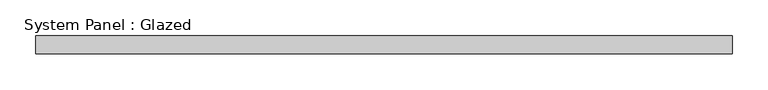
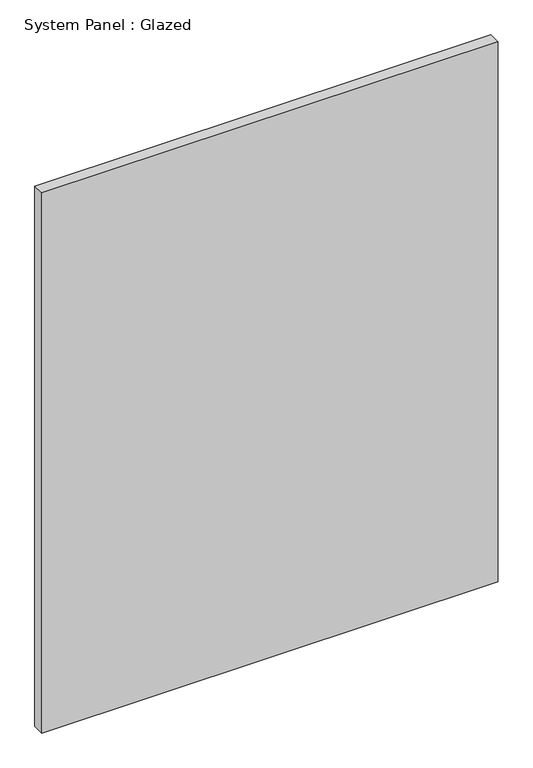
"""IFC4 building model written with IfcOpenShell, lengths in millimetres: plate geometry, System Panel : Glazed."""

import ifcopenshell
import ifcopenshell.guid

model = None  # the IFC model being written
_history = None  # IfcOwnerHistory: only IFC2X3 demands one
_inside = {}  # id of a spatial element -> (the spatial element, [elements in it])
_under = {}  # id of a project, library or spatial element -> (it, [spatial elements below it])
_declared = {}  # id of a project -> (the project, [libraries it declares])
_typed = {}  # id of a type object -> (the type object, [elements of that type])
_made_of = {}  # id of a material, layer set ... -> (it, [elements and type objects made of it])


def new_model(schema):
    """Start an empty IFC model of exactly this schema.

    Asked for "IFC4X3", IfcOpenShell would pick the latest addendum, in which some entities
    have other attributes; the version numbers below select the first issue.
    IFC2X3 requires an IfcOwnerHistory on every rooted entity: one is made here for all.
    """
    global model, _history
    if schema == "IFC4X3":
        model = ifcopenshell.file(schema_version=(4, 3, 0, 0))
    else:
        model = ifcopenshell.file(schema=schema)
    _inside.clear()
    _under.clear()
    _declared.clear()
    _typed.clear()
    _made_of.clear()
    _history = None
    if model.schema == "IFC2X3":
        org = make("IfcOrganization", Name="unknown")
        user = make(
            "IfcPersonAndOrganization",
            ThePerson=make("IfcPerson", FamilyName="unknown"),
            TheOrganization=org,
        )
        app = make(
            "IfcApplication",
            ApplicationDeveloper=org,
            Version="unknown",
            ApplicationFullName="unknown",
            ApplicationIdentifier="unknown",
        )
        _history = make(
            "IfcOwnerHistory",
            OwningUser=user,
            OwningApplication=app,
            ChangeAction="ADDED",
            CreationDate=0,
        )
    return model


def make(cls, **values):
    """One entity of the class cls with the attributes given. An attribute that is None is left unset."""
    return model.create_entity(
        cls, **{name: value for name, value in values.items() if value is not None}
    )


def rooted(cls, **values):
    """An entity with a GlobalId (a new one), such as an element, a storey or a relation."""
    return make(cls, GlobalId=ifcopenshell.guid.new(), OwnerHistory=_history, **values)


def si_unit(unit_type, name, prefix=None):
    """IfcSIUnit, for example si_unit("LENGTHUNIT", "METRE", prefix="MILLI")."""
    return make("IfcSIUnit", UnitType=unit_type, Prefix=prefix, Name=name)


def assignment(units):
    """IfcUnitAssignment: the units of a project."""
    return None if units is None else make("IfcUnitAssignment", Units=units)


def point(xyz):
    """IfcCartesianPoint."""
    return None if xyz is None else make("IfcCartesianPoint", Coordinates=xyz)


def direction(xyz):
    """IfcDirection."""
    return None if xyz is None else make("IfcDirection", DirectionRatios=xyz)


def frame(location, z_axis=None, x_axis=None):
    """IfcAxis2Placement3D, a coordinate frame: its origin and axes. An axis left out is left unset."""
    return make(
        "IfcAxis2Placement3D",
        Location=point(location),
        Axis=direction(z_axis),
        RefDirection=direction(x_axis),
    )


def origin():
    """The frame at (0, 0, 0) with its axes left unset."""
    return frame((0.0, 0.0, 0.0))


def origin_with_axes():
    """The frame at (0, 0, 0) with the z axis (0, 0, 1) and the x axis (1, 0, 0) written out."""
    return frame((0.0, 0.0, 0.0), z_axis=(0.0, 0.0, 1.0), x_axis=(1.0, 0.0, 0.0))


def place(relative_to, where):
    """IfcLocalPlacement: puts the frame where relative to a parent placement (None: the world)."""
    return make(
        "IfcLocalPlacement", PlacementRelTo=relative_to, RelativePlacement=where
    )


def context(
    kind, dimensions, precision=None, world=None, true_north=None, identifier=None
):
    """IfcGeometricRepresentationContext, for example the 3D "Model" context."""
    return make(
        "IfcGeometricRepresentationContext",
        ContextIdentifier=identifier,
        ContextType=kind,
        CoordinateSpaceDimension=dimensions,
        Precision=precision,
        WorldCoordinateSystem=world,
        TrueNorth=true_north,
    )


def project(units=None, contexts=None):
    """IfcProject with its units and contexts."""
    return rooted(
        "IfcProject",
        Name="project",
        RepresentationContexts=contexts,
        UnitsInContext=assignment(units),
    )


def spatial(cls, under=None, at=None, **own):
    """A site, building, storey or space (cls), placed at a placement, below another one or the project."""
    s = rooted(cls, ObjectPlacement=at, **own)
    if under is not None:
        _under.setdefault(under.id(), (under, []))[1].append(s)
    return s


def polyline(points):
    """IfcPolyline through the points."""
    return make("IfcPolyline", Points=[point(p) for p in points])


def outline(outer, holes=None, kind="AREA"):
    """IfcArbitraryClosedProfileDef: a profile drawn as a closed curve; with holes, ...WithVoids."""
    if holes is None:
        return make("IfcArbitraryClosedProfileDef", ProfileType=kind, OuterCurve=outer)
    return make(
        "IfcArbitraryProfileDefWithVoids",
        ProfileType=kind,
        OuterCurve=outer,
        InnerCurves=holes,
    )


def extrude(swept, where, along, depth):
    """IfcExtrudedAreaSolid: the profile swept, set in the frame where, extruded along a direction by depth."""
    return make(
        "IfcExtrudedAreaSolid",
        SweptArea=swept,
        Position=where,
        ExtrudedDirection=direction(along),
        Depth=depth,
    )


def shape(context_of_items, identifier, shape_type, items):
    """IfcShapeRepresentation: the items that make up one representation, for example the "Body"."""
    return make(
        "IfcShapeRepresentation",
        ContextOfItems=context_of_items,
        RepresentationIdentifier=identifier,
        RepresentationType=shape_type,
        Items=items,
    )


def source(mapping_origin, context_of_items, identifier, shape_type, items):
    """IfcRepresentationMap: a shape defined once, which mapped items show again and again."""
    return make(
        "IfcRepresentationMap",
        MappingOrigin=mapping_origin,
        MappedRepresentation=shape(context_of_items, identifier, shape_type, items),
    )


def transform(
    local_origin,
    x_axis=None,
    y_axis=None,
    z_axis=None,
    scale=None,
    scale2=None,
    scale3=None,
    uniform=True,
):
    """IfcCartesianTransformationOperator3D, or its non-uniform kind. x_axis, y_axis, z_axis: its Axis1, 2, 3."""
    if uniform:
        return make(
            "IfcCartesianTransformationOperator3D",
            Axis1=direction(x_axis),
            Axis2=direction(y_axis),
            LocalOrigin=point(local_origin),
            Scale=scale,
            Axis3=direction(z_axis),
        )
    return make(
        "IfcCartesianTransformationOperator3DnonUniform",
        Axis1=direction(x_axis),
        Axis2=direction(y_axis),
        LocalOrigin=point(local_origin),
        Scale=scale,
        Axis3=direction(z_axis),
        Scale2=scale2,
        Scale3=scale3,
    )


def mapped(mapping_source, mapping_target):
    """IfcMappedItem: shows the shape of a source again, moved by a transform."""
    return make(
        "IfcMappedItem", MappingSource=mapping_source, MappingTarget=mapping_target
    )


def made_of(thing, what):
    """Note that an element or type object is made of a material, layer set ...; save() writes the relation."""
    if what is not None:
        _made_of.setdefault(what.id(), (what, []))[1].append(thing)
    return thing


def element(
    cls,
    number,
    at=None,
    inside=None,
    cuts=None,
    type_object=None,
    material=None,
    context=None,
    identifier="Body",
    shape_type=None,
    held_by="IfcProductDefinitionShape",
    body=None,
    shapes=None,
    **own,
):
    """One element of the class cls, such as IfcWall. Its Tag is "e" and its number.

    at: its placement. inside: the storey or other place that contains it. cuts: it is an
    opening in that element (IfcRelVoidsElement). A single representation is given by context,
    identifier, shape_type and body (its items); several are given by shapes. held_by: the class
    of the entity that holds the representations. save() writes the other relations.
    """
    e = rooted(cls, Tag="e%d" % number, ObjectPlacement=at, **own)
    if body is not None:
        shapes = [shape(context, identifier, shape_type, body)]
    if shapes is not None:
        e.Representation = make(held_by, Representations=shapes)
    if inside is not None:
        _inside.setdefault(inside.id(), (inside, []))[1].append(e)
    if cuts is not None:
        rooted(
            "IfcRelVoidsElement", RelatingBuildingElement=cuts, RelatedOpeningElement=e
        )
    if type_object is not None:
        _typed.setdefault(type_object.id(), (type_object, []))[1].append(e)
    return made_of(e, material)


def aggregate(whole, parts):
    """IfcRelAggregates: a whole, such as a stair, and the parts it consists of."""
    return rooted("IfcRelAggregates", RelatingObject=whole, RelatedObjects=parts)


def save(model, path):
    """Write the relations noted so far, then the file.

    IfcRelAggregates (storeys below a building ...), IfcRelContainedInSpatialStructure (elements
    in a storey), IfcRelDefinesByType, IfcRelAssociatesMaterial and IfcRelDeclares: one each for
    every whole, place, type object, material and project.
    """
    for whole, parts in _under.values():
        aggregate(whole, parts)
    for where, things in _inside.values():
        rooted(
            "IfcRelContainedInSpatialStructure",
            RelatedElements=things,
            RelatingStructure=where,
        )
    for kind, things in _typed.values():
        rooted("IfcRelDefinesByType", RelatedObjects=things, RelatingType=kind)
    for what, things in _made_of.values():
        rooted("IfcRelAssociatesMaterial", RelatedObjects=things, RelatingMaterial=what)
    for by, libraries in _declared.values():
        rooted("IfcRelDeclares", RelatingContext=by, RelatedDefinitions=libraries)
    model.write(path)


def system_panel_glazed_f71ae7e5(model_context):
    return source(origin(), model_context, "Body", "SweptSolid", [
        extrude(outline(polyline([(487.1405982, -44.45), (-487.1405982, -44.45), (-487.1405982, -19.05), (487.1405982, -19.05), (487.1405982, -44.45)])), origin_with_axes(), (0.0, 0.0, 1.0), 1219.2),
    ])


if __name__ == "__main__":
    model = new_model("IFC4")
    model_context = context("Model", 3, world=origin())
    ifc_project = project(units=[si_unit("LENGTHUNIT", "METRE", prefix="MILLI")], contexts=[model_context])
    site = spatial("IfcSite", under=ifc_project)
    building = spatial("IfcBuilding", under=site)
    placement = place(None, origin())
    system_panel_glazed_shape = system_panel_glazed_f71ae7e5(model_context)
    element("IfcPlate", 1, ObjectType="System Panel : Glazed", at=placement, inside=building, context=model_context, shape_type="MappedRepresentation", body=[
        mapped(system_panel_glazed_shape, transform((0.0, 0.0, 0.0), x_axis=(1.0, 0.0, 0.0), y_axis=(0.0, 1.0, 0.0), z_axis=(0.0, 0.0, 1.0))),
    ])
    save(model, "model.ifc")

# Revit data of these elements
# Element 1 (IfcPlate, "System Panel : Glazed")
#   Materials on its faces: "Glass"
# Materials
#   "Glass": class "Glass", colour RGB 0 128 192, transparency 0.75
